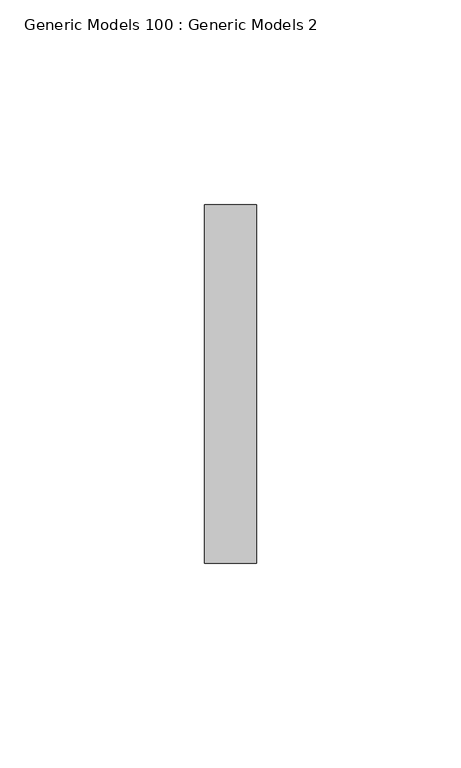
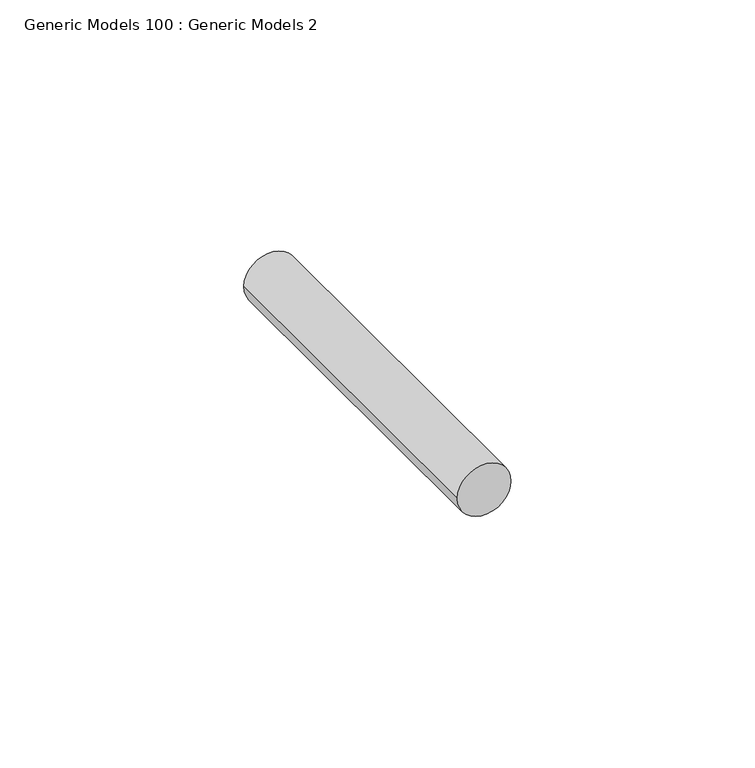
"""IFC4 building model written with IfcOpenShell, lengths in millimetres: proxy geometry, Generic Models 100 : Generic Models 2."""

from ifc_helpers import new_model, si_unit, point, frame, frame_2d, origin, place, context, project, spatial, circle_curve, trimmed, segment, composite_curve, outline, extrude, source, transform, mapped, element, save


def generic_models_100_generic_models_2_0454f8a4(model_context):
    return source(origin(), model_context, "Body", "SweptSolid", [
        extrude(outline(composite_curve([segment(trimmed(circle_curve(frame_2d((37174.3647633, 5621.1346014)), 6.35), [point((37174.3647633, 5627.4846014))], [point((37174.3647633, 5614.7846014))], False, "CARTESIAN"), True, "CONTINUOUS"), segment(trimmed(circle_curve(frame_2d((37174.3647633, 5621.1346014)), 6.35), [point((37174.3647633, 5614.7846014))], [point((37174.3647633, 5627.4846014))], False, "CARTESIAN"), True, "CONTINUOUS")], self_intersect=False)), frame((0.0, 1848.3666731, 0.0), z_axis=(0.0, 1.0, 0.0), x_axis=(0.0, 0.0, 1.0)), (0.0, 0.0, 1.0), 87.551022),
    ])


if __name__ == "__main__":
    model = new_model("IFC4")
    model_context = context("Model", 3, world=origin())
    ifc_project = project(units=[si_unit("LENGTHUNIT", "METRE", prefix="MILLI")], contexts=[model_context])
    site = spatial("IfcSite", under=ifc_project)
    building = spatial("IfcBuilding", under=site)
    placement = place(None, origin())
    generic_models_100_generic_models_2_shape = generic_models_100_generic_models_2_0454f8a4(model_context)
    element("IfcBuildingElementProxy", 1, Name="Generic Models 100 : Generic Models 2", ObjectType="Generic Models 100 : Generic Models 2", at=placement, inside=building, context=model_context, shape_type="MappedRepresentation", body=[
        mapped(generic_models_100_generic_models_2_shape, transform((0.0, 0.0, 0.0), x_axis=(1.0, 0.0, 0.0), y_axis=(0.0, 1.0, 0.0), z_axis=(0.0, 0.0, 1.0))),
    ])
    save(model, "model.ifc")

# Revit data of these elements
# Element 1 (IfcBuildingElementProxy, "Generic Models 100 : Generic Models 2")
#   Materials on its faces: "S.S. LAG BOLT - SEE STRUCT. DWGS"
# Materials
#   "S.S. LAG BOLT - SEE STRUCT. DWGS": class "Generic", colour RGB 120 120 120, transparency 0, Cost = 0
